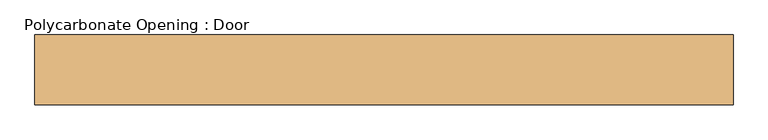
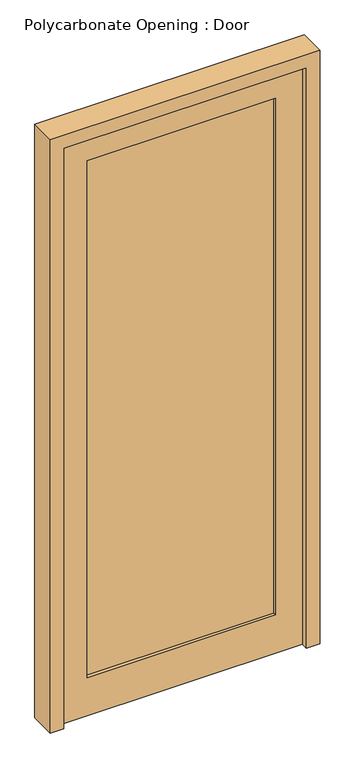
"""IFC4 building model written with IfcOpenShell, lengths in millimetres: door geometry, Polycarbonate Opening : Door."""

from ifc_helpers import new_model, si_unit, frame, origin, place, context, project, spatial, polyline, outline, extrude, source, transform, mapped, element, save


def polycarbonate_opening_door_e1fcdb3c(model_context):
    return source(origin(), model_context, "Body", "SweptSolid", [
        extrude(outline(polyline([(457.2, 0.0), (-457.2, 0.0), (-457.2, 25.4), (457.2, 25.4), (457.2, 0.0)])), frame((0.0, 0.0, 50.8), z_axis=(0.0, 0.0, 1.0), x_axis=(1.0, 0.0, 0.0)), (0.0, 0.0, 1.0), 2260.6),
        extrude(outline(polyline([(2311.4, -457.2), (0.0, -457.2), (0.0, 457.2), (2311.4, 457.2), (2311.4, -457.2)]), holes=[polyline([(152.4, 355.6), (152.4, -355.6), (2209.8, -355.6), (2209.8, 355.6), (152.4, 355.6)])]), frame((0.0, -12.7, 0.0), z_axis=(0.0, 1.0, 0.0), x_axis=(0.0, 0.0, 1.0)), (0.0, 0.0, 1.0), 50.8),
        extrude(outline(polyline([(2362.2, 508.0), (2362.2, -508.0), (0.0, -508.0), (0.0, -457.2), (2311.4, -457.2), (2311.4, 457.2), (0.0, 457.2), (0.0, 508.0), (2362.2, 508.0)])), frame((0.0, -38.1, 0.0), z_axis=(0.0, 1.0, 0.0), x_axis=(0.0, 0.0, 1.0)), (0.0, 0.0, 1.0), 101.6),
    ])


if __name__ == "__main__":
    model = new_model("IFC4")
    model_context = context("Model", 3, world=origin())
    ifc_project = project(units=[si_unit("LENGTHUNIT", "METRE", prefix="MILLI")], contexts=[model_context])
    site = spatial("IfcSite", under=ifc_project)
    building = spatial("IfcBuilding", under=site)
    placement = place(None, origin())
    polycarbonate_opening_door_shape = polycarbonate_opening_door_e1fcdb3c(model_context)
    element("IfcDoor", 1, ObjectType="Polycarbonate Opening : Door", at=placement, inside=building, context=model_context, shape_type="MappedRepresentation", body=[
        mapped(polycarbonate_opening_door_shape, transform((0.0, 0.0, 0.0), x_axis=(1.0, 0.0, 0.0), y_axis=(0.0, 1.0, 0.0), z_axis=(0.0, 0.0, 1.0))),
    ])
    save(model, "model.ifc")

# Revit data of these elements
# Type "Polycarbonate Opening : Door"
#   Type Mark = "60"
#   Analytic Construction = "<None>"
#   offset [instance default] = 0' - 0 1/2"
#   Stile = 0' - 4"
#   Mullion Width = 0' - 2"
#   Mullion Depth = 0' - 4"
#   Opening Size [instance default] = 5' - 1.50212"
#   Door Width [instance default] = 5' - 1.50212"
#   Window ON/OFF = yes
#   Door On/Off = no
#   Mullion Material = ALUMINUM STOREFRONT
#   Glass Material = INSULATED GLAZING
#   Door Material = ALUMINUM STOREFRONT
# Element 1 (IfcDoor, "Polycarbonate Opening : Door")
#   Materials on its faces: "ALUMINUM STOREFRONT", "INSULATED GLAZING"
# Materials
#   "ALUMINUM STOREFRONT": class "Metal", colour RGB 244 244 244, transparency 0, Description = "Aluminum 6061", Cost = 0
#   "INSULATED GLAZING": class "Glass", colour RGB 196 205 210, transparency 0.85, Description = "Soda Lime Glass", Cost = 0
